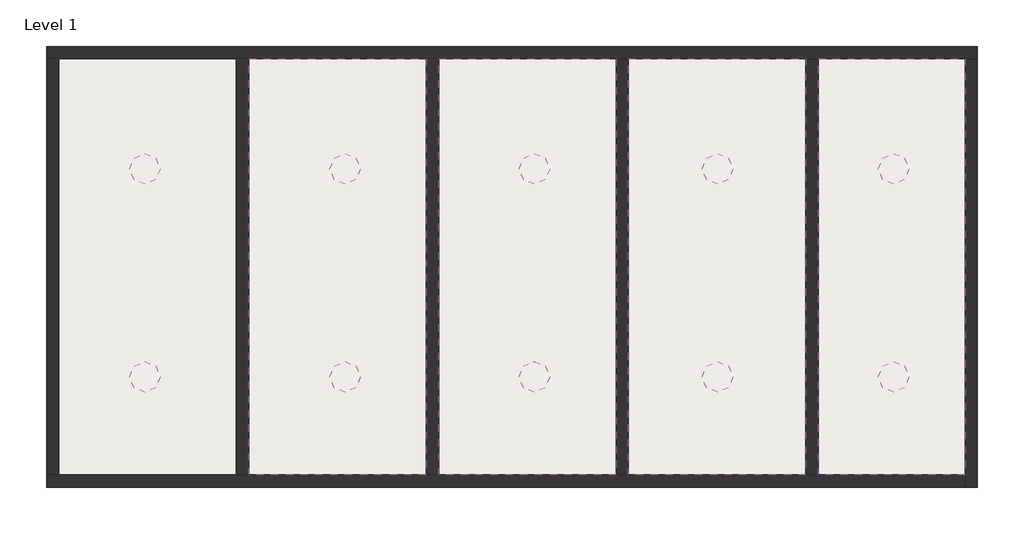
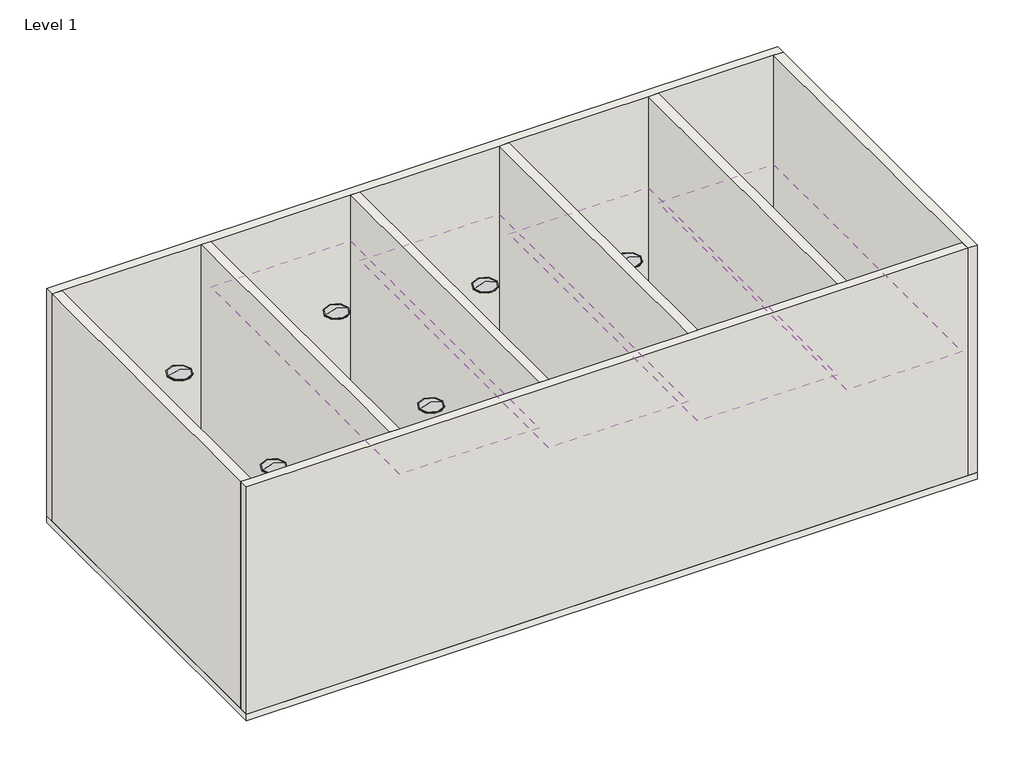
# One storey: 10 light fixtures, 8 walls, 4 coverings, 1 slab.
"""IFC4 building model written with IfcOpenShell, lengths in millimetres."""

import ifcopenshell
import ifcopenshell.guid

model = None  # the IFC model being written
_history = None  # IfcOwnerHistory: only IFC2X3 demands one
_inside = {}  # id of a spatial element -> (the spatial element, [elements in it])
_under = {}  # id of a project, library or spatial element -> (it, [spatial elements below it])
_declared = {}  # id of a project -> (the project, [libraries it declares])
_typed = {}  # id of a type object -> (the type object, [elements of that type])
_made_of = {}  # id of a material, layer set ... -> (it, [elements and type objects made of it])


def new_model(schema):
    """Start an empty IFC model of exactly this schema.

    Asked for "IFC4X3", IfcOpenShell would pick the latest addendum, in which some entities
    have other attributes; the version numbers below select the first issue.
    IFC2X3 requires an IfcOwnerHistory on every rooted entity: one is made here for all.
    """
    global model, _history
    if schema == "IFC4X3":
        model = ifcopenshell.file(schema_version=(4, 3, 0, 0))
    else:
        model = ifcopenshell.file(schema=schema)
    _inside.clear()
    _under.clear()
    _declared.clear()
    _typed.clear()
    _made_of.clear()
    _history = None
    if model.schema == "IFC2X3":
        org = make("IfcOrganization", Name="unknown")
        user = make(
            "IfcPersonAndOrganization",
            ThePerson=make("IfcPerson", FamilyName="unknown"),
            TheOrganization=org,
        )
        app = make(
            "IfcApplication",
            ApplicationDeveloper=org,
            Version="unknown",
            ApplicationFullName="unknown",
            ApplicationIdentifier="unknown",
        )
        _history = make(
            "IfcOwnerHistory",
            OwningUser=user,
            OwningApplication=app,
            ChangeAction="ADDED",
            CreationDate=0,
        )
    return model


def make(cls, **values):
    """One entity of the class cls with the attributes given. An attribute that is None is left unset."""
    return model.create_entity(
        cls, **{name: value for name, value in values.items() if value is not None}
    )


def rooted(cls, **values):
    """An entity with a GlobalId (a new one), such as an element, a storey or a relation."""
    return make(cls, GlobalId=ifcopenshell.guid.new(), OwnerHistory=_history, **values)


def si_unit(unit_type, name, prefix=None):
    """IfcSIUnit, for example si_unit("LENGTHUNIT", "METRE", prefix="MILLI")."""
    return make("IfcSIUnit", UnitType=unit_type, Prefix=prefix, Name=name)


def assignment(units):
    """IfcUnitAssignment: the units of a project."""
    return None if units is None else make("IfcUnitAssignment", Units=units)


def point(xyz):
    """IfcCartesianPoint."""
    return None if xyz is None else make("IfcCartesianPoint", Coordinates=xyz)


def direction(xyz):
    """IfcDirection."""
    return None if xyz is None else make("IfcDirection", DirectionRatios=xyz)


def frame(location, z_axis=None, x_axis=None):
    """IfcAxis2Placement3D, a coordinate frame: its origin and axes. An axis left out is left unset."""
    return make(
        "IfcAxis2Placement3D",
        Location=point(location),
        Axis=direction(z_axis),
        RefDirection=direction(x_axis),
    )


def frame_2d(location, x_axis=None):
    """IfcAxis2Placement2D, a coordinate frame in the plane: its origin and x axis."""
    return make(
        "IfcAxis2Placement2D", Location=point(location), RefDirection=direction(x_axis)
    )


def origin():
    """The frame at (0, 0, 0) with its axes left unset."""
    return frame((0.0, 0.0, 0.0))


def origin_with_axes():
    """The frame at (0, 0, 0) with the z axis (0, 0, 1) and the x axis (1, 0, 0) written out."""
    return frame((0.0, 0.0, 0.0), z_axis=(0.0, 0.0, 1.0), x_axis=(1.0, 0.0, 0.0))


def origin_2d():
    """The frame at (0, 0) in the plane with its x axis left unset."""
    return frame_2d((0.0, 0.0))


def place(relative_to, where):
    """IfcLocalPlacement: puts the frame where relative to a parent placement (None: the world)."""
    return make(
        "IfcLocalPlacement", PlacementRelTo=relative_to, RelativePlacement=where
    )


def context(
    kind, dimensions, precision=None, world=None, true_north=None, identifier=None
):
    """IfcGeometricRepresentationContext, for example the 3D "Model" context."""
    return make(
        "IfcGeometricRepresentationContext",
        ContextIdentifier=identifier,
        ContextType=kind,
        CoordinateSpaceDimension=dimensions,
        Precision=precision,
        WorldCoordinateSystem=world,
        TrueNorth=true_north,
    )


def project(units=None, contexts=None):
    """IfcProject with its units and contexts."""
    return rooted(
        "IfcProject",
        Name="project",
        RepresentationContexts=contexts,
        UnitsInContext=assignment(units),
    )


def spatial(cls, under=None, at=None, **own):
    """A site, building, storey or space (cls), placed at a placement, below another one or the project."""
    s = rooted(cls, ObjectPlacement=at, **own)
    if under is not None:
        _under.setdefault(under.id(), (under, []))[1].append(s)
    return s


def polyline(points):
    """IfcPolyline through the points."""
    return make("IfcPolyline", Points=[point(p) for p in points])


def circle_curve(where, radius):
    """IfcCircle in the frame where."""
    return make("IfcCircle", Position=where, Radius=radius)


def ellipse_curve(where, semi_axis1, semi_axis2):
    """IfcEllipse in the frame where."""
    return make(
        "IfcEllipse", Position=where, SemiAxis1=semi_axis1, SemiAxis2=semi_axis2
    )


def trimmed(basis, trim1, trim2, sense, master):
    """IfcTrimmedCurve: the piece of a basis curve between two trims."""
    return make(
        "IfcTrimmedCurve",
        BasisCurve=basis,
        Trim1=trim1,
        Trim2=trim2,
        SenseAgreement=sense,
        MasterRepresentation=master,
    )


def segment(curve, same_sense, transition):
    """IfcCompositeCurveSegment."""
    return make(
        "IfcCompositeCurveSegment",
        Transition=transition,
        SameSense=same_sense,
        ParentCurve=curve,
    )


def composite_curve(segments, self_intersect=None):
    """IfcCompositeCurve: segments joined end to end."""
    return make("IfcCompositeCurve", Segments=segments, SelfIntersect=self_intersect)


def outline(outer, holes=None, kind="AREA"):
    """IfcArbitraryClosedProfileDef: a profile drawn as a closed curve; with holes, ...WithVoids."""
    if holes is None:
        return make("IfcArbitraryClosedProfileDef", ProfileType=kind, OuterCurve=outer)
    return make(
        "IfcArbitraryProfileDefWithVoids",
        ProfileType=kind,
        OuterCurve=outer,
        InnerCurves=holes,
    )


def extrude(swept, where, along, depth):
    """IfcExtrudedAreaSolid: the profile swept, set in the frame where, extruded along a direction by depth."""
    return make(
        "IfcExtrudedAreaSolid",
        SweptArea=swept,
        Position=where,
        ExtrudedDirection=direction(along),
        Depth=depth,
    )


def faces_of(points, faces, orient=None, outer=None):
    """IfcFace entities. A face is a list of loops; a loop is a list of indices into points, from 0.

    orient and outer hold one flag for each loop. By default every Orientation is true, the
    first loop of a face is its IfcFaceOuterBound and the others are IfcFaceBound.
    """
    made = []
    for i, loops in enumerate(faces):
        bounds = []
        for j, loop in enumerate(loops):
            is_outer = j == 0 if outer is None else outer[i][j]
            bounds.append(
                make(
                    "IfcFaceOuterBound" if is_outer else "IfcFaceBound",
                    Bound=make("IfcPolyLoop", Polygon=[points[k] for k in loop]),
                    Orientation=True if orient is None else orient[i][j],
                )
            )
        made.append(make("IfcFace", Bounds=bounds))
    return made


def faceted_brep(points, faces, orient=None, outer=None, voids=None):
    """IfcFacetedBrep: a solid bounded by flat faces; with voids (closed shells), ...WithVoids."""
    shared = [point(p) for p in points]
    hull = make("IfcClosedShell", CfsFaces=faces_of(shared, faces, orient, outer))
    if voids is None:
        return make("IfcFacetedBrep", Outer=hull)
    return make(
        "IfcFacetedBrepWithVoids",
        Outer=hull,
        Voids=[
            make(cls, CfsFaces=faces_of(shared, fs, o, b)) for cls, fs, o, b in voids
        ],
    )


def shape(context_of_items, identifier, shape_type, items):
    """IfcShapeRepresentation: the items that make up one representation, for example the "Body"."""
    return make(
        "IfcShapeRepresentation",
        ContextOfItems=context_of_items,
        RepresentationIdentifier=identifier,
        RepresentationType=shape_type,
        Items=items,
    )


def source(mapping_origin, context_of_items, identifier, shape_type, items):
    """IfcRepresentationMap: a shape defined once, which mapped items show again and again."""
    return make(
        "IfcRepresentationMap",
        MappingOrigin=mapping_origin,
        MappedRepresentation=shape(context_of_items, identifier, shape_type, items),
    )


def transform(
    local_origin,
    x_axis=None,
    y_axis=None,
    z_axis=None,
    scale=None,
    scale2=None,
    scale3=None,
    uniform=True,
):
    """IfcCartesianTransformationOperator3D, or its non-uniform kind. x_axis, y_axis, z_axis: its Axis1, 2, 3."""
    if uniform:
        return make(
            "IfcCartesianTransformationOperator3D",
            Axis1=direction(x_axis),
            Axis2=direction(y_axis),
            LocalOrigin=point(local_origin),
            Scale=scale,
            Axis3=direction(z_axis),
        )
    return make(
        "IfcCartesianTransformationOperator3DnonUniform",
        Axis1=direction(x_axis),
        Axis2=direction(y_axis),
        LocalOrigin=point(local_origin),
        Scale=scale,
        Axis3=direction(z_axis),
        Scale2=scale2,
        Scale3=scale3,
    )


def mapped(mapping_source, mapping_target):
    """IfcMappedItem: shows the shape of a source again, moved by a transform."""
    return make(
        "IfcMappedItem", MappingSource=mapping_source, MappingTarget=mapping_target
    )


def made_of(thing, what):
    """Note that an element or type object is made of a material, layer set ...; save() writes the relation."""
    if what is not None:
        _made_of.setdefault(what.id(), (what, []))[1].append(thing)
    return thing


def element(
    cls,
    number,
    at=None,
    inside=None,
    cuts=None,
    type_object=None,
    material=None,
    context=None,
    identifier="Body",
    shape_type=None,
    held_by="IfcProductDefinitionShape",
    body=None,
    shapes=None,
    **own,
):
    """One element of the class cls, such as IfcWall. Its Tag is "e" and its number.

    at: its placement. inside: the storey or other place that contains it. cuts: it is an
    opening in that element (IfcRelVoidsElement). A single representation is given by context,
    identifier, shape_type and body (its items); several are given by shapes. held_by: the class
    of the entity that holds the representations. save() writes the other relations.
    """
    e = rooted(cls, Tag="e%d" % number, ObjectPlacement=at, **own)
    if body is not None:
        shapes = [shape(context, identifier, shape_type, body)]
    if shapes is not None:
        e.Representation = make(held_by, Representations=shapes)
    if inside is not None:
        _inside.setdefault(inside.id(), (inside, []))[1].append(e)
    if cuts is not None:
        rooted(
            "IfcRelVoidsElement", RelatingBuildingElement=cuts, RelatedOpeningElement=e
        )
    if type_object is not None:
        _typed.setdefault(type_object.id(), (type_object, []))[1].append(e)
    return made_of(e, material)


def aggregate(whole, parts):
    """IfcRelAggregates: a whole, such as a stair, and the parts it consists of."""
    return rooted("IfcRelAggregates", RelatingObject=whole, RelatedObjects=parts)


def save(model, path):
    """Write the relations noted so far, then the file.

    IfcRelAggregates (storeys below a building ...), IfcRelContainedInSpatialStructure (elements
    in a storey), IfcRelDefinesByType, IfcRelAssociatesMaterial and IfcRelDeclares: one each for
    every whole, place, type object, material and project.
    """
    for whole, parts in _under.values():
        aggregate(whole, parts)
    for where, things in _inside.values():
        rooted(
            "IfcRelContainedInSpatialStructure",
            RelatedElements=things,
            RelatingStructure=where,
        )
    for kind, things in _typed.values():
        rooted("IfcRelDefinesByType", RelatedObjects=things, RelatingType=kind)
    for what, things in _made_of.values():
        rooted("IfcRelAssociatesMaterial", RelatedObjects=things, RelatingMaterial=what)
    for by, libraries in _declared.values():
        rooted("IfcRelDeclares", RelatingContext=by, RelatedDefinitions=libraries)
    model.write(path)


def plane_surface(at):
    """IfcPlane: the flat surface through the origin of the frame at, square to its z axis."""
    return make("IfcPlane", Position=at)


def revolved_surface(curve, axis_point, axis_direction):
    """IfcSurfaceOfRevolution: the curve turned about the line through axis_point along axis_direction."""
    return make(
        "IfcSurfaceOfRevolution",
        SweptCurve=make("IfcArbitraryOpenProfileDef", ProfileType="CURVE", Curve=curve),
        AxisPosition=make("IfcAxis1Placement", Location=point(axis_point), Axis=direction(axis_direction)),
    )


def advanced_brep(points, edges, surfaces, faces):
    """IfcAdvancedBrep: a solid bounded by faces that lie on surfaces and meet in shared edges.

    An edge is (start, end): straight between two places in points (the first is 0);
    or (start, end, curve); or (start, end, curve, False) where it runs against its curve.
    A face is (place in surfaces, loops), or (place, loops, False) where it looks against
    its surface's normal. A loop lists edges by number (the first is 1), with a minus sign
    where the edge is run from its end to its start. The first loop is the outer one.
    """
    corners = [point(p) for p in points]
    vertices = [make("IfcVertexPoint", VertexGeometry=c) for c in corners]
    made = []
    for start, end, *more in edges:
        made.append(
            make(
                "IfcEdgeCurve",
                EdgeStart=vertices[start],
                EdgeEnd=vertices[end],
                EdgeGeometry=more[0] if more else make("IfcPolyline", Points=[corners[start], corners[end]]),
                SameSense=more[1] if len(more) > 1 else True,
            )
        )
    hull = []
    for where, loops, *sense in faces:
        bounds = []
        for j, loop in enumerate(loops):
            ring = [make("IfcOrientedEdge", EdgeElement=made[abs(k) - 1], Orientation=k > 0) for k in loop]
            bounds.append(
                make(
                    "IfcFaceOuterBound" if j == 0 else "IfcFaceBound",
                    Bound=make("IfcEdgeLoop", EdgeList=ring),
                    Orientation=True,
                )
            )
        hull.append(make("IfcAdvancedFace", Bounds=bounds, FaceSurface=surfaces[where], SameSense=sense[0] if sense else True))
    return make("IfcAdvancedBrep", Outer=make("IfcClosedShell", CfsFaces=hull))


def downlight_downlight_e6a68a7d(model_context):
    return source(origin(), model_context, "Body", "SolidModel", [
        advanced_brep(
        [(-230.0, 0.0, 0.0), (230.0, 0.0, 0.0), (0.0, 0.0, 0.0), (0.0, 0.0, 70.3180567)],
        [
            (0, 1, circle_curve(frame((0.0, 0.0, 0.0), z_axis=(0.0, 0.0, -1.0), x_axis=(1.0, 0.0, 0.0)), 230.0)),
            (1, 2),
            (2, 0),
            (1, 0, circle_curve(frame((0.0, 0.0, 0.0), z_axis=(0.0, 0.0, -1.0), x_axis=(1.0, 0.0, 0.0)), 230.0)),
            (3, 1, circle_curve(frame((13.1969865, 0.0, -297.8236248), z_axis=(0.0, 1.0, 0.0), x_axis=(1.0, 0.0, 0.0)), 368.3781456)),
            (0, 3, circle_curve(frame((-13.1969865, 0.0, -297.8236248), z_axis=(0.0, 1.0, 0.0), x_axis=(-1.0, 0.0, 0.0)), 368.3781456)),
        ],
        [
            plane_surface(frame((0.0, 0.0, 0.0), z_axis=(0.0, 0.0, -1.0), x_axis=(1.0, 0.0, 0.0))),
            revolved_surface(trimmed(ellipse_curve(frame((13.1969865, 0.0, -297.8236248), z_axis=(0.0, -1.0, 0.0), x_axis=(1.0, 0.0, 0.0)), 368.3781456, 368.3781456), [point((230.0, 0.0, 0.0))], [point((0.0, 0.0, 70.3180567))], True, "CARTESIAN"), (0.0, 0.0, 2194.0651339), (0.0, 0.0, 1.0)),
        ],
        [
            (0, [[1, 2, 3]]),
            (0, [[4, -3, -2]]),
            (1, [[5, -1, 6]]),
            (1, [[-6, -4, -5]]),
        ],
    ),
        extrude(outline(composite_curve([segment(trimmed(circle_curve(origin_2d(), 250.0), [point((-250.0, 0.0))], [point((250.0, 0.0))], False, "CARTESIAN"), True, "CONTINUOUS"), segment(trimmed(circle_curve(origin_2d(), 250.0), [point((250.0, 0.0))], [point((-250.0, 0.0))], False, "CARTESIAN"), True, "CONTINUOUS")], self_intersect=False)), frame((0.0, 0.0, -10.1537533), z_axis=(0.0, 0.0, 1.0), x_axis=(1.0, 0.0, 0.0)), (0.0, 0.0, 1.0), 10.1537533),
    ])


model = new_model("IFC4")

# Units and contexts
model_context = context("Model", 3, world=origin())
ifc_project = project(units=[si_unit("LENGTHUNIT", "METRE", prefix="MILLI")], contexts=[model_context])

# Site, building, storey
site = spatial("IfcSite", under=ifc_project)
building = spatial("IfcBuilding", under=site)
storey = spatial("IfcBuildingStorey", under=building, Name="Level 1", Elevation=0.0)

# Coverings
placement = place(None, origin())
element("IfcCovering", 1, ObjectType="Plain", at=placement, inside=storey, context=model_context, shape_type="SweptSolid", body=[
    extrude(outline(polyline([(4711.6370984, -2494.7382368), (4711.6370984, 4305.2617632), (7111.6370984, 4305.2617632), (7111.6370984, -2494.7382368), (4711.6370984, -2494.7382368)])), frame((0.0, 0.0, 2600.0), z_axis=(0.0, 0.0, 1.0), x_axis=(1.0, 0.0, 0.0)), (0.0, 0.0, 1.0), 57.0),
])
element("IfcCovering", 2, ObjectType="Plain", at=placement, inside=storey, context=model_context, shape_type="SweptSolid", body=[
    extrude(outline(polyline([(1611.6370984, -2494.7382368), (1611.6370984, 4305.2617632), (4511.6370984, 4305.2617632), (4511.6370984, -2494.7382368), (1611.6370984, -2494.7382368)])), frame((0.0, 0.0, 3000.0), z_axis=(0.0, 0.0, 1.0), x_axis=(1.0, 0.0, 0.0)), (0.0, 0.0, 1.0), 57.0),
])
element("IfcCovering", 3, ObjectType="Plain", at=placement, inside=storey, context=model_context, shape_type="SweptSolid", body=[
    extrude(outline(polyline([(-1488.3629016, -2494.7382368), (-1488.3629016, 4305.2617632), (1411.6370984, 4305.2617632), (1411.6370984, -2494.7382368), (-1488.3629016, -2494.7382368)])), frame((0.0, 0.0, 3500.0), z_axis=(0.0, 0.0, 1.0), x_axis=(1.0, 0.0, 0.0)), (0.0, 0.0, 1.0), 57.0),
])
element("IfcCovering", 4, ObjectType="Plain", at=placement, inside=storey, context=model_context, shape_type="SweptSolid", body=[
    extrude(outline(polyline([(-4588.3629016, -2494.7382368), (-4588.3629016, 4305.2617632), (-1688.3629016, 4305.2617632), (-1688.3629016, -2494.7382368), (-4588.3629016, -2494.7382368)])), frame((0.0, 0.0, 4000.0), z_axis=(0.0, 0.0, 1.0), x_axis=(1.0, 0.0, 0.0)), (0.0, 0.0, 1.0), 57.0),
])

# Light fixtures
downlight_downlight_shape = downlight_downlight_e6a68a7d(model_context)
element("IfcLightFixture", 5, ObjectType="Downlight : Downlight", at=placement, inside=storey, context=model_context, shape_type="MappedRepresentation", body=[
    mapped(downlight_downlight_shape, transform((-6282.0675101, -895.1572455, 3800.0), x_axis=(1.0, 0.0, 0.0), y_axis=(0.0, 1.0, 0.0), z_axis=(0.0, 0.0, 1.0))),
])
element("IfcLightFixture", 6, ObjectType="Downlight : Downlight", at=placement, inside=storey, context=model_context, shape_type="MappedRepresentation", body=[
    mapped(downlight_downlight_shape, transform((-6282.0675101, 2504.8427545, 3800.0), x_axis=(1.0, 0.0, 0.0), y_axis=(0.0, 1.0, 0.0), z_axis=(0.0, 0.0, 1.0))),
])
element("IfcLightFixture", 7, ObjectType="Downlight : Downlight", at=placement, inside=storey, context=model_context, shape_type="MappedRepresentation", body=[
    mapped(downlight_downlight_shape, transform((-3013.7777439, -895.1572455, 4000.0), x_axis=(1.0, 0.0, 0.0), y_axis=(0.0, 1.0, 0.0), z_axis=(0.0, 0.0, 1.0))),
])
element("IfcLightFixture", 8, ObjectType="Downlight : Downlight", at=placement, inside=storey, context=model_context, shape_type="MappedRepresentation", body=[
    mapped(downlight_downlight_shape, transform((-3013.7777439, 2504.8427545, 4000.0), x_axis=(1.0, 0.0, 0.0), y_axis=(0.0, 1.0, 0.0), z_axis=(0.0, 0.0, 1.0))),
])
element("IfcLightFixture", 9, ObjectType="Downlight : Downlight", at=placement, inside=storey, context=model_context, shape_type="MappedRepresentation", body=[
    mapped(downlight_downlight_shape, transform((76.5388311, -895.1572455, 3500.0), x_axis=(1.0, 0.0, 0.0), y_axis=(0.0, 1.0, 0.0), z_axis=(0.0, 0.0, 1.0))),
])
element("IfcLightFixture", 10, ObjectType="Downlight : Downlight", at=placement, inside=storey, context=model_context, shape_type="MappedRepresentation", body=[
    mapped(downlight_downlight_shape, transform((76.5388311, 2504.8427545, 3500.0), x_axis=(1.0, 0.0, 0.0), y_axis=(0.0, 1.0, 0.0), z_axis=(0.0, 0.0, 1.0))),
])
element("IfcLightFixture", 11, ObjectType="Downlight : Downlight", at=placement, inside=storey, context=model_context, shape_type="MappedRepresentation", body=[
    mapped(downlight_downlight_shape, transform((3067.3545284, -895.1572455, 3000.0), x_axis=(1.0, 0.0, 0.0), y_axis=(0.0, 1.0, 0.0), z_axis=(0.0, 0.0, 1.0))),
])
element("IfcLightFixture", 12, ObjectType="Downlight : Downlight", at=placement, inside=storey, context=model_context, shape_type="MappedRepresentation", body=[
    mapped(downlight_downlight_shape, transform((3067.3545284, 2504.8427545, 3000.0), x_axis=(1.0, 0.0, 0.0), y_axis=(0.0, 1.0, 0.0), z_axis=(0.0, 0.0, 1.0))),
])
element("IfcLightFixture", 13, ObjectType="Downlight : Downlight", at=placement, inside=storey, context=model_context, shape_type="MappedRepresentation", body=[
    mapped(downlight_downlight_shape, transform((5942.4423645, -895.1572455, 2600.0), x_axis=(1.0, 0.0, 0.0), y_axis=(0.0, 1.0, 0.0), z_axis=(0.0, 0.0, 1.0))),
])
element("IfcLightFixture", 14, ObjectType="Downlight : Downlight", at=placement, inside=storey, context=model_context, shape_type="MappedRepresentation", body=[
    mapped(downlight_downlight_shape, transform((5942.4423645, 2504.8427545, 2600.0), x_axis=(1.0, 0.0, 0.0), y_axis=(0.0, 1.0, 0.0), z_axis=(0.0, 0.0, 1.0))),
])

# Slab
element("IfcSlab", 15, ObjectType="Generic 150mm", at=placement, inside=storey, context=model_context, shape_type="SweptSolid", body=[
    extrude(outline(polyline([(7311.6370984, 4505.2617632), (7311.6370984, -2694.7382368), (-7888.3629016, -2694.7382368), (-7888.3629016, 4505.2617632), (7311.6370984, 4505.2617632)])), frame((0.0, 0.0, -150.0), z_axis=(0.0, 0.0, 1.0), x_axis=(1.0, 0.0, 0.0)), (0.0, 0.0, 1.0), 150.0),
])

# Walls
element("IfcWall", 16, ObjectType="Generic - 200mm", at=placement, inside=storey, context=model_context, shape_type="Brep", body=[
    faceted_brep([(-7888.3629016, 4305.2617632, 0.0), (-7688.3629016, 4305.2617632, 0.0), (-4788.3629016, 4305.2617632, 0.0), (-4588.3629016, 4305.2617632, 0.0), (-1688.3629016, 4305.2617632, 0.0), (-1488.3629016, 4305.2617632, 0.0), (1411.6370984, 4305.2617632, 0.0), (1611.6370984, 4305.2617632, 0.0), (4511.6370984, 4305.2617632, 0.0), (4711.6370984, 4305.2617632, 0.0), (7111.6370984, 4305.2617632, 0.0), (7311.6370984, 4305.2617632, 0.0), (7311.6370984, 4305.2617632, 5000.0), (7111.6370984, 4305.2617632, 5000.0), (4711.6370984, 4305.2617632, 5000.0), (4511.6370984, 4305.2617632, 5000.0), (1611.6370984, 4305.2617632, 5000.0), (1411.6370984, 4305.2617632, 5000.0), (-1488.3629016, 4305.2617632, 5000.0), (-1688.3629016, 4305.2617632, 5000.0), (-4588.3629016, 4305.2617632, 5000.0), (-4788.3629016, 4305.2617632, 5000.0), (-7688.3629016, 4305.2617632, 5000.0), (-7888.3629016, 4305.2617632, 5000.0), (-7888.3629016, 4505.2617632, 0.0), (-7888.3629016, 4505.2617632, 5000.0), (7311.6370984, 4505.2617632, 5000.0), (7311.6370984, 4505.2617632, 0.0)], [[[0, 1, 2, 3, 4, 5, 6, 7, 8, 9, 10, 11, 12, 13, 14, 15, 16, 17, 18, 19, 20, 21, 22, 23]], [[24, 25, 26, 27]], [[11, 10, 9, 8, 7, 6, 5, 4, 3, 2, 1, 0, 24, 27]], [[23, 22, 21, 20, 19, 18, 17, 16, 15, 14, 13, 12, 26, 25]], [[12, 11, 27, 26]], [[0, 23, 25, 24]]]),
])
element("IfcWall", 17, ObjectType="Generic - 200mm", at=placement, inside=storey, context=model_context, shape_type="Brep", body=[
    faceted_brep([(7111.6370984, 4305.2617632, 0.0), (7111.6370984, -2494.7382368, 0.0), (7111.6370984, -2694.7382368, 0.0), (7111.6370984, -2694.7382368, 5000.0), (7111.6370984, -2494.7382368, 5000.0), (7111.6370984, 4305.2617632, 5000.0), (7311.6370984, 4305.2617632, 0.0), (7311.6370984, 4305.2617632, 5000.0), (7311.6370984, -2694.7382368, 5000.0), (7311.6370984, -2694.7382368, 0.0)], [[[0, 1, 2, 3, 4, 5]], [[6, 7, 8, 9]], [[2, 1, 0, 6, 9]], [[5, 4, 3, 8, 7]], [[0, 5, 7, 6]], [[3, 2, 9, 8]]]),
])
element("IfcWall", 18, ObjectType="Generic - 200mm", at=placement, inside=storey, context=model_context, shape_type="Brep", body=[
    faceted_brep([(7111.6370984, -2494.7382368, 0.0), (4711.6370984, -2494.7382368, 0.0), (4511.6370984, -2494.7382368, 0.0), (1611.6370984, -2494.7382368, 0.0), (1411.6370984, -2494.7382368, 0.0), (-1488.3629016, -2494.7382368, 0.0), (-1688.3629016, -2494.7382368, 0.0), (-4588.3629016, -2494.7382368, 0.0), (-4788.3629016, -2494.7382368, 0.0), (-7688.3629016, -2494.7382368, 0.0), (-7888.3629016, -2494.7382368, 0.0), (-7888.3629016, -2494.7382368, 5000.0), (-7688.3629016, -2494.7382368, 5000.0), (-4788.3629016, -2494.7382368, 5000.0), (-4588.3629016, -2494.7382368, 5000.0), (-1688.3629016, -2494.7382368, 5000.0), (-1488.3629016, -2494.7382368, 5000.0), (1411.6370984, -2494.7382368, 5000.0), (1611.6370984, -2494.7382368, 5000.0), (4511.6370984, -2494.7382368, 5000.0), (4711.6370984, -2494.7382368, 5000.0), (7111.6370984, -2494.7382368, 5000.0), (7111.6370984, -2694.7382368, 0.0), (7111.6370984, -2694.7382368, 5000.0), (-7888.3629016, -2694.7382368, 5000.0), (-7888.3629016, -2694.7382368, 0.0)], [[[0, 1, 2, 3, 4, 5, 6, 7, 8, 9, 10, 11, 12, 13, 14, 15, 16, 17, 18, 19, 20, 21]], [[22, 23, 24, 25]], [[10, 9, 8, 7, 6, 5, 4, 3, 2, 1, 0, 22, 25]], [[21, 20, 19, 18, 17, 16, 15, 14, 13, 12, 11, 24, 23]], [[0, 21, 23, 22]], [[11, 10, 25, 24]]]),
])
element("IfcWall", 19, ObjectType="Generic - 200mm", at=placement, inside=storey, context=model_context, shape_type="SweptSolid", body=[
    extrude(outline(polyline([(-7688.3629016, 4305.2617632), (-7688.3629016, -2494.7382368), (-7888.3629016, -2494.7382368), (-7888.3629016, 4305.2617632), (-7688.3629016, 4305.2617632)])), origin_with_axes(), (0.0, 0.0, 1.0), 5000.0),
])
element("IfcWall", 20, ObjectType="Generic - 200mm", at=placement, inside=storey, context=model_context, shape_type="SweptSolid", body=[
    extrude(outline(polyline([(-4788.3629016, -2494.7382368), (-4788.3629016, 4305.2617632), (-4588.3629016, 4305.2617632), (-4588.3629016, -2494.7382368), (-4788.3629016, -2494.7382368)])), origin_with_axes(), (0.0, 0.0, 1.0), 5000.0),
])
element("IfcWall", 21, ObjectType="Generic - 200mm", at=placement, inside=storey, context=model_context, shape_type="SweptSolid", body=[
    extrude(outline(polyline([(-1688.3629016, -2494.7382368), (-1688.3629016, 4305.2617632), (-1488.3629016, 4305.2617632), (-1488.3629016, -2494.7382368), (-1688.3629016, -2494.7382368)])), origin_with_axes(), (0.0, 0.0, 1.0), 5000.0),
])
element("IfcWall", 22, ObjectType="Generic - 200mm", at=placement, inside=storey, context=model_context, shape_type="SweptSolid", body=[
    extrude(outline(polyline([(1411.6370984, -2494.7382368), (1411.6370984, 4305.2617632), (1611.6370984, 4305.2617632), (1611.6370984, -2494.7382368), (1411.6370984, -2494.7382368)])), origin_with_axes(), (0.0, 0.0, 1.0), 5000.0),
])
element("IfcWall", 23, ObjectType="Generic - 200mm", at=placement, inside=storey, context=model_context, shape_type="SweptSolid", body=[
    extrude(outline(polyline([(4511.6370984, -2494.7382368), (4511.6370984, 4305.2617632), (4711.6370984, 4305.2617632), (4711.6370984, -2494.7382368), (4511.6370984, -2494.7382368)])), origin_with_axes(), (0.0, 0.0, 1.0), 5000.0),
])

save(model, "model.ifc")

# Revit data of these elements
# Project information
#   Project Issue Date = "Issue Date"
#   Project Status = "Project Status"
#   Client Name = "Owner"
#   Project Address = "Enter address here"
#   Project Name = "Project Name"
#   Project Number = "0001"
# Type "Plain"
#   built-in parameter 1002203 = 1 (stored number, unit not read)
#   built-in parameter 1002202 = 1 (stored number, unit not read)
#   Layers, outside or top first: 0.045 m "Metal Stud Layer" (function 1); 0.012 m "Gypsum Wall Board" (function 1)
# Type "Downlight : Downlight"
#   Default Elevation = 0
# Type "Generic 150mm"
#   Function = 0
#   Layers, outside or top first: 0.15 m no material (function 1)
# Type "Generic - 200mm"
#   Layers, outside or top first: 0.2 m no material (function 1)
# Element 1 (IfcCovering, "Plain")
#   Height Offset From Level = 2.6 m
#   Phase Created = New Construction
#   Materials on its faces: "Gypsum Wall Board", "Metal Stud Layer"
# Element 2 (IfcCovering, "Plain")
#   Height Offset From Level = 3 m
#   Phase Created = New Construction
#   Materials on its faces: "Gypsum Wall Board", "Metal Stud Layer"
# Element 3 (IfcCovering, "Plain")
#   Height Offset From Level = 3.5 m
#   Phase Created = New Construction
#   Materials on its faces: "Gypsum Wall Board", "Metal Stud Layer"
# Element 4 (IfcCovering, "Plain")
#   Height Offset From Level = 4 m
#   Phase Created = New Construction
#   Materials on its faces: "Gypsum Wall Board", "Metal Stud Layer"
# Element 5 (IfcLightFixture, "Downlight : Downlight")
#   Mark = "23"
#   Phase Created = New Construction
# Element 6 (IfcLightFixture, "Downlight : Downlight")
#   Mark = "24"
#   Phase Created = New Construction
# Element 7 (IfcLightFixture, "Downlight : Downlight")
#   Mark = "25"
#   Phase Created = New Construction
# Element 8 (IfcLightFixture, "Downlight : Downlight")
#   Mark = "26"
#   Phase Created = New Construction
# Element 9 (IfcLightFixture, "Downlight : Downlight")
#   Mark = "27"
#   Phase Created = New Construction
# Element 10 (IfcLightFixture, "Downlight : Downlight")
#   Mark = "28"
#   Phase Created = New Construction
# Element 11 (IfcLightFixture, "Downlight : Downlight")
#   Mark = "29"
#   Phase Created = New Construction
# Element 12 (IfcLightFixture, "Downlight : Downlight")
#   Mark = "30"
#   Phase Created = New Construction
# Element 13 (IfcLightFixture, "Downlight : Downlight")
#   Mark = "31"
#   Phase Created = New Construction
# Element 14 (IfcLightFixture, "Downlight : Downlight")
#   Mark = "32"
#   Phase Created = New Construction
# Element 15 (IfcSlab, "Generic 150mm")
#   Height Offset From Level = 0 m
#   Phase Created = New Construction
#   Materials on its faces: "Default Floor"
# Elements 16, 17, 18, 19, 20, 21, 22, 23 (IfcWall, "Generic - 200mm")
#   Top Offset = 0 m
#   Base Offset = 0 m
#   wall height = 5 m
#   Phase Created = New Construction
#   Base Constraint = Level 1
#   Top Constraint = Level 2
#   Materials on its faces: "Default Wall"
# Materials
#   "Metal Stud Layer": class "Metal", colour RGB 127 127 127, transparency 0, Description = "Light gauge steel framing, thermal air layer", Cost = 0
#   "Gypsum Wall Board": class "Generic", colour RGB 249 249 249, transparency 0, Description = "Gypsum Wall Board", Cost = 0
#   "Default Floor": class "Miscellaneous", colour RGB 127 127 127, transparency 0, Cost = 0
#   "Default Wall": class "Miscellaneous", colour RGB 128 128 128, transparency 0, Cost = 0
